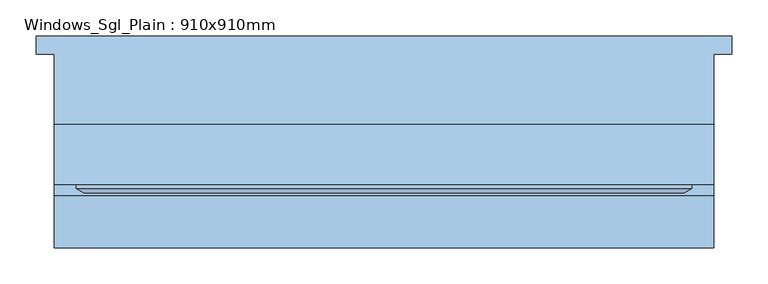
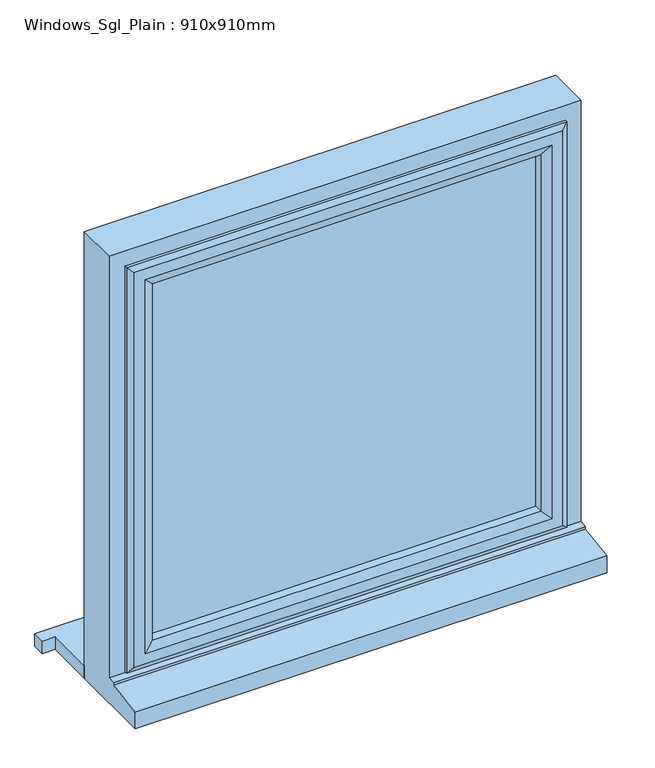
"""IFC4 building model written with IfcOpenShell, lengths in millimetres: window geometry, Windows_Sgl_Plain : 910x910mm."""

import ifcopenshell
import ifcopenshell.guid

model = None  # the IFC model being written
_history = None  # IfcOwnerHistory: only IFC2X3 demands one
_inside = {}  # id of a spatial element -> (the spatial element, [elements in it])
_under = {}  # id of a project, library or spatial element -> (it, [spatial elements below it])
_declared = {}  # id of a project -> (the project, [libraries it declares])
_typed = {}  # id of a type object -> (the type object, [elements of that type])
_made_of = {}  # id of a material, layer set ... -> (it, [elements and type objects made of it])


def new_model(schema):
    """Start an empty IFC model of exactly this schema.

    Asked for "IFC4X3", IfcOpenShell would pick the latest addendum, in which some entities
    have other attributes; the version numbers below select the first issue.
    IFC2X3 requires an IfcOwnerHistory on every rooted entity: one is made here for all.
    """
    global model, _history
    if schema == "IFC4X3":
        model = ifcopenshell.file(schema_version=(4, 3, 0, 0))
    else:
        model = ifcopenshell.file(schema=schema)
    _inside.clear()
    _under.clear()
    _declared.clear()
    _typed.clear()
    _made_of.clear()
    _history = None
    if model.schema == "IFC2X3":
        org = make("IfcOrganization", Name="unknown")
        user = make(
            "IfcPersonAndOrganization",
            ThePerson=make("IfcPerson", FamilyName="unknown"),
            TheOrganization=org,
        )
        app = make(
            "IfcApplication",
            ApplicationDeveloper=org,
            Version="unknown",
            ApplicationFullName="unknown",
            ApplicationIdentifier="unknown",
        )
        _history = make(
            "IfcOwnerHistory",
            OwningUser=user,
            OwningApplication=app,
            ChangeAction="ADDED",
            CreationDate=0,
        )
    return model


def make(cls, **values):
    """One entity of the class cls with the attributes given. An attribute that is None is left unset."""
    return model.create_entity(
        cls, **{name: value for name, value in values.items() if value is not None}
    )


def rooted(cls, **values):
    """An entity with a GlobalId (a new one), such as an element, a storey or a relation."""
    return make(cls, GlobalId=ifcopenshell.guid.new(), OwnerHistory=_history, **values)


def si_unit(unit_type, name, prefix=None):
    """IfcSIUnit, for example si_unit("LENGTHUNIT", "METRE", prefix="MILLI")."""
    return make("IfcSIUnit", UnitType=unit_type, Prefix=prefix, Name=name)


def assignment(units):
    """IfcUnitAssignment: the units of a project."""
    return None if units is None else make("IfcUnitAssignment", Units=units)


def point(xyz):
    """IfcCartesianPoint."""
    return None if xyz is None else make("IfcCartesianPoint", Coordinates=xyz)


def direction(xyz):
    """IfcDirection."""
    return None if xyz is None else make("IfcDirection", DirectionRatios=xyz)


def frame(location, z_axis=None, x_axis=None):
    """IfcAxis2Placement3D, a coordinate frame: its origin and axes. An axis left out is left unset."""
    return make(
        "IfcAxis2Placement3D",
        Location=point(location),
        Axis=direction(z_axis),
        RefDirection=direction(x_axis),
    )


def origin():
    """The frame at (0, 0, 0) with its axes left unset."""
    return frame((0.0, 0.0, 0.0))


def place(relative_to, where):
    """IfcLocalPlacement: puts the frame where relative to a parent placement (None: the world)."""
    return make(
        "IfcLocalPlacement", PlacementRelTo=relative_to, RelativePlacement=where
    )


def context(
    kind, dimensions, precision=None, world=None, true_north=None, identifier=None
):
    """IfcGeometricRepresentationContext, for example the 3D "Model" context."""
    return make(
        "IfcGeometricRepresentationContext",
        ContextIdentifier=identifier,
        ContextType=kind,
        CoordinateSpaceDimension=dimensions,
        Precision=precision,
        WorldCoordinateSystem=world,
        TrueNorth=true_north,
    )


def project(units=None, contexts=None):
    """IfcProject with its units and contexts."""
    return rooted(
        "IfcProject",
        Name="project",
        RepresentationContexts=contexts,
        UnitsInContext=assignment(units),
    )


def spatial(cls, under=None, at=None, **own):
    """A site, building, storey or space (cls), placed at a placement, below another one or the project."""
    s = rooted(cls, ObjectPlacement=at, **own)
    if under is not None:
        _under.setdefault(under.id(), (under, []))[1].append(s)
    return s


def polyline(points):
    """IfcPolyline through the points."""
    return make("IfcPolyline", Points=[point(p) for p in points])


def outline(outer, holes=None, kind="AREA"):
    """IfcArbitraryClosedProfileDef: a profile drawn as a closed curve; with holes, ...WithVoids."""
    if holes is None:
        return make("IfcArbitraryClosedProfileDef", ProfileType=kind, OuterCurve=outer)
    return make(
        "IfcArbitraryProfileDefWithVoids",
        ProfileType=kind,
        OuterCurve=outer,
        InnerCurves=holes,
    )


def extrude(swept, where, along, depth):
    """IfcExtrudedAreaSolid: the profile swept, set in the frame where, extruded along a direction by depth."""
    return make(
        "IfcExtrudedAreaSolid",
        SweptArea=swept,
        Position=where,
        ExtrudedDirection=direction(along),
        Depth=depth,
    )


def faces_of(points, faces, orient=None, outer=None):
    """IfcFace entities. A face is a list of loops; a loop is a list of indices into points, from 0.

    orient and outer hold one flag for each loop. By default every Orientation is true, the
    first loop of a face is its IfcFaceOuterBound and the others are IfcFaceBound.
    """
    made = []
    for i, loops in enumerate(faces):
        bounds = []
        for j, loop in enumerate(loops):
            is_outer = j == 0 if outer is None else outer[i][j]
            bounds.append(
                make(
                    "IfcFaceOuterBound" if is_outer else "IfcFaceBound",
                    Bound=make("IfcPolyLoop", Polygon=[points[k] for k in loop]),
                    Orientation=True if orient is None else orient[i][j],
                )
            )
        made.append(make("IfcFace", Bounds=bounds))
    return made


def faceted_brep(points, faces, orient=None, outer=None, voids=None):
    """IfcFacetedBrep: a solid bounded by flat faces; with voids (closed shells), ...WithVoids."""
    shared = [point(p) for p in points]
    hull = make("IfcClosedShell", CfsFaces=faces_of(shared, faces, orient, outer))
    if voids is None:
        return make("IfcFacetedBrep", Outer=hull)
    return make(
        "IfcFacetedBrepWithVoids",
        Outer=hull,
        Voids=[
            make(cls, CfsFaces=faces_of(shared, fs, o, b)) for cls, fs, o, b in voids
        ],
    )


def shape(context_of_items, identifier, shape_type, items):
    """IfcShapeRepresentation: the items that make up one representation, for example the "Body"."""
    return make(
        "IfcShapeRepresentation",
        ContextOfItems=context_of_items,
        RepresentationIdentifier=identifier,
        RepresentationType=shape_type,
        Items=items,
    )


def source(mapping_origin, context_of_items, identifier, shape_type, items):
    """IfcRepresentationMap: a shape defined once, which mapped items show again and again."""
    return make(
        "IfcRepresentationMap",
        MappingOrigin=mapping_origin,
        MappedRepresentation=shape(context_of_items, identifier, shape_type, items),
    )


def transform(
    local_origin,
    x_axis=None,
    y_axis=None,
    z_axis=None,
    scale=None,
    scale2=None,
    scale3=None,
    uniform=True,
):
    """IfcCartesianTransformationOperator3D, or its non-uniform kind. x_axis, y_axis, z_axis: its Axis1, 2, 3."""
    if uniform:
        return make(
            "IfcCartesianTransformationOperator3D",
            Axis1=direction(x_axis),
            Axis2=direction(y_axis),
            LocalOrigin=point(local_origin),
            Scale=scale,
            Axis3=direction(z_axis),
        )
    return make(
        "IfcCartesianTransformationOperator3DnonUniform",
        Axis1=direction(x_axis),
        Axis2=direction(y_axis),
        LocalOrigin=point(local_origin),
        Scale=scale,
        Axis3=direction(z_axis),
        Scale2=scale2,
        Scale3=scale3,
    )


def mapped(mapping_source, mapping_target):
    """IfcMappedItem: shows the shape of a source again, moved by a transform."""
    return make(
        "IfcMappedItem", MappingSource=mapping_source, MappingTarget=mapping_target
    )


def made_of(thing, what):
    """Note that an element or type object is made of a material, layer set ...; save() writes the relation."""
    if what is not None:
        _made_of.setdefault(what.id(), (what, []))[1].append(thing)
    return thing


def element(
    cls,
    number,
    at=None,
    inside=None,
    cuts=None,
    type_object=None,
    material=None,
    context=None,
    identifier="Body",
    shape_type=None,
    held_by="IfcProductDefinitionShape",
    body=None,
    shapes=None,
    **own,
):
    """One element of the class cls, such as IfcWall. Its Tag is "e" and its number.

    at: its placement. inside: the storey or other place that contains it. cuts: it is an
    opening in that element (IfcRelVoidsElement). A single representation is given by context,
    identifier, shape_type and body (its items); several are given by shapes. held_by: the class
    of the entity that holds the representations. save() writes the other relations.
    """
    e = rooted(cls, Tag="e%d" % number, ObjectPlacement=at, **own)
    if body is not None:
        shapes = [shape(context, identifier, shape_type, body)]
    if shapes is not None:
        e.Representation = make(held_by, Representations=shapes)
    if inside is not None:
        _inside.setdefault(inside.id(), (inside, []))[1].append(e)
    if cuts is not None:
        rooted(
            "IfcRelVoidsElement", RelatingBuildingElement=cuts, RelatedOpeningElement=e
        )
    if type_object is not None:
        _typed.setdefault(type_object.id(), (type_object, []))[1].append(e)
    return made_of(e, material)


def aggregate(whole, parts):
    """IfcRelAggregates: a whole, such as a stair, and the parts it consists of."""
    return rooted("IfcRelAggregates", RelatingObject=whole, RelatedObjects=parts)


def save(model, path):
    """Write the relations noted so far, then the file.

    IfcRelAggregates (storeys below a building ...), IfcRelContainedInSpatialStructure (elements
    in a storey), IfcRelDefinesByType, IfcRelAssociatesMaterial and IfcRelDeclares: one each for
    every whole, place, type object, material and project.
    """
    for whole, parts in _under.values():
        aggregate(whole, parts)
    for where, things in _inside.values():
        rooted(
            "IfcRelContainedInSpatialStructure",
            RelatedElements=things,
            RelatingStructure=where,
        )
    for kind, things in _typed.values():
        rooted("IfcRelDefinesByType", RelatedObjects=things, RelatingType=kind)
    for what, things in _made_of.values():
        rooted("IfcRelAssociatesMaterial", RelatedObjects=things, RelatingMaterial=what)
    for by, libraries in _declared.values():
        rooted("IfcRelDeclares", RelatingContext=by, RelatedDefinitions=libraries)
    model.write(path)


def windows_sgl_plain_910x910mm_d8acfbc0(model_context):
    return source(origin(), model_context, "Body", "SolidModel", [
        extrude(outline(polyline([(-480.0, 131.5434322), (480.0, 131.5434322), (480.0, 106.5434322), (455.0, 106.5434322), (455.0, 9.5434322), (-455.0, 9.5434322), (-455.0, 106.5434322), (-480.0, 106.5434322), (-480.0, 131.5434322)])), frame((0.0, 0.0, 1200.0), z_axis=(0.0, 0.0, 1.0), x_axis=(1.0, 0.0, 0.0)), (0.0, 0.0, 1.0), 25.0),
        faceted_brep([(-455.0, 9.5434322, 1200.0), (-455.0, 9.5434322, 2110.0), (455.0, 9.5434322, 2110.0), (455.0, 9.5434322, 1200.0), (-395.0, 9.5434322, 2050.0), (-395.0, 9.5434322, 1275.0), (395.0, 9.5434322, 1275.0), (395.0, 9.5434322, 2050.0), (-455.0, -160.9565678, 1200.0), (-455.0, -160.9565678, 1233.8088847), (-455.0, -88.4565678, 1244.7449676), (-455.0, -88.4565678, 1249.68767), (-455.0, -73.4565678, 1251.0), (-455.0, -73.4565678, 2110.0), (455.0, -73.4565678, 1251.0), (455.0, -73.4565678, 2110.0), (-415.0, -73.4565678, 2070.0), (415.0, -73.4565678, 2070.0), (415.0, -73.4565678, 1263.0), (-415.0, -73.4565678, 1263.0), (-415.0, -8.4565678, 1263.0), (-415.0, -8.4565678, 2070.0), (415.0, -8.4565678, 1263.0), (415.0, -8.4565678, 2070.0), (-395.0, -8.4565678, 2050.0), (395.0, -8.4565678, 2050.0), (395.0, -8.4565678, 1275.0), (-395.0, -8.4565678, 1275.0), (455.0, -88.4565678, 1249.68767), (455.0, -88.4565678, 1244.7449676), (455.0, -160.9565678, 1233.8088847), (455.0, -160.9565678, 1200.0)], [[[0, 1, 2, 3], [4, 5, 6, 7]], [[0, 8, 9, 10, 11, 12, 13, 1]], [[12, 14, 15, 13], [16, 17, 18, 19]], [[19, 20, 21, 16]], [[21, 20, 22, 23], [24, 25, 26, 27]], [[24, 27, 5, 4]], [[1, 13, 15, 2]], [[16, 21, 23, 17]], [[7, 25, 24, 4]], [[14, 28, 29, 30, 31, 3, 2, 15]], [[17, 23, 22, 18]], [[7, 6, 26, 25]], [[31, 8, 0, 3]], [[30, 9, 8, 31]], [[29, 10, 9, 30]], [[28, 11, 10, 29]], [[14, 12, 11, 28]], [[20, 19, 18, 22]], [[5, 27, 26, 6]]]),
        extrude(outline(polyline([(385.0, -37.4565678), (385.0, -61.4565678), (-385.0, -61.4565678), (-385.0, -37.4565678), (385.0, -37.4565678)])), frame((0.0, 0.0, 1293.0), z_axis=(0.0, 0.0, 1.0), x_axis=(1.0, 0.0, 0.0)), (0.0, 0.0, 1.0), 747.0),
        faceted_brep([(-425.0, -73.4565678, 2080.0), (-425.0, -73.4565678, 1253.0), (-425.0, -79.2300705, 1253.0), (-425.0, -79.2300705, 2080.0), (-415.0, -8.4565678, 2070.0), (-415.0, -8.4565678, 1263.0), (-415.0, -73.4565678, 1263.0), (-415.0, -73.4565678, 2070.0), (-375.0, -22.9494677, 2030.0), (-375.0, -22.9494677, 1303.0), (-385.1480377, -8.4565678, 1292.8519623), (-385.1480377, -8.4565678, 2040.1480377), (-375.0, -37.4565678, 2030.0), (-375.0, -37.4565678, 1303.0), (-385.0, -61.4565678, 2040.0), (-385.0, -61.4565678, 1293.0), (-385.0, -37.4565678, 1293.0), (-385.0, -37.4565678, 2040.0), (-375.0, -79.2300705, 2030.0), (-375.0, -79.2300705, 1303.0), (-375.0, -61.4565678, 1303.0), (-375.0, -61.4565678, 2030.0), (-392.4457548, -85.0035732, 2047.4457548), (-392.4457548, -85.0035732, 1285.5542452), (-414.2153903, -85.0035732, 1263.7846097), (-414.2153903, -85.0035732, 2069.2153903), (425.0, -73.4565678, 1253.0), (425.0, -79.2300705, 1253.0), (415.0, -8.4565678, 1263.0), (415.0, -73.4565678, 1263.0), (375.0, -22.9494677, 1303.0), (385.1480377, -8.4565678, 1292.8519623), (375.0, -37.4565678, 1303.0), (385.0, -61.4565678, 1293.0), (385.0, -37.4565678, 1293.0), (375.0, -79.2300705, 1303.0), (375.0, -61.4565678, 1303.0), (392.4457548, -85.0035732, 1285.5542452), (414.2153903, -85.0035732, 1263.7846097), (425.0, -73.4565678, 2080.0), (425.0, -79.2300705, 2080.0), (415.0, -8.4565678, 2070.0), (415.0, -73.4565678, 2070.0), (375.0, -22.9494677, 2030.0), (385.1480377, -8.4565678, 2040.1480377), (375.0, -37.4565678, 2030.0), (385.0, -61.4565678, 2040.0), (385.0, -37.4565678, 2040.0), (375.0, -79.2300705, 2030.0), (375.0, -61.4565678, 2030.0), (392.4457548, -85.0035732, 2047.4457548), (414.2153903, -85.0035732, 2069.2153903)], [[[0, 1, 2, 3]], [[4, 5, 6, 7]], [[8, 9, 10, 11]], [[12, 13, 9, 8]], [[14, 15, 16, 17]], [[18, 19, 20, 21]], [[22, 23, 19, 18]], [[3, 2, 24, 25]], [[1, 26, 27, 2]], [[5, 28, 29, 6]], [[9, 30, 31, 10]], [[13, 32, 30, 9]], [[15, 33, 34, 16]], [[19, 35, 36, 20]], [[23, 37, 35, 19]], [[2, 27, 38, 24]], [[26, 39, 40, 27]], [[28, 41, 42, 29]], [[30, 43, 44, 31]], [[32, 45, 43, 30]], [[33, 46, 47, 34]], [[35, 48, 49, 36]], [[37, 50, 48, 35]], [[27, 40, 51, 38]], [[39, 0, 3, 40]], [[1, 0, 39, 26], [7, 6, 29, 42]], [[41, 4, 7, 42]], [[5, 4, 41, 28], [11, 10, 31, 44]], [[43, 8, 11, 44]], [[45, 12, 8, 43]], [[17, 16, 34, 47], [13, 12, 45, 32]], [[46, 14, 17, 47]], [[15, 14, 46, 33], [21, 20, 36, 49]], [[48, 18, 21, 49]], [[50, 22, 18, 48]], [[25, 24, 38, 51], [23, 22, 50, 37]], [[40, 3, 25, 51]]]),
    ])


if __name__ == "__main__":
    model = new_model("IFC4")
    model_context = context("Model", 3, world=origin())
    ifc_project = project(units=[si_unit("LENGTHUNIT", "METRE", prefix="MILLI")], contexts=[model_context])
    site = spatial("IfcSite", under=ifc_project)
    building = spatial("IfcBuilding", under=site)
    placement = place(None, origin())
    windows_sgl_plain_910x910mm_shape = windows_sgl_plain_910x910mm_d8acfbc0(model_context)
    element("IfcWindow", 1, ObjectType="Windows_Sgl_Plain : 910x910mm", at=placement, inside=building, context=model_context, shape_type="MappedRepresentation", body=[
        mapped(windows_sgl_plain_910x910mm_shape, transform((0.0, 0.0, 0.0), x_axis=(1.0, 0.0, 0.0), y_axis=(0.0, 1.0, 0.0), z_axis=(0.0, 0.0, 1.0))),
    ])
    save(model, "model.ifc")

# Revit data of these elements
# Type "Windows_Sgl_Plain : 910x910mm"
#   Type Mark = "44"
#   Operation = "SinglePanel"
#   Construction Type Id = "SGL"
#   Manufacturer = "Revit"
#   Keynote = "L10"
#   Analytic Construction = "Large single-glazed windows"
#   Wrap Layers (Ext) from Ext = 102.5 mm
#   Wrap Layers (Int) from Ext = 177.5 mm
#   Window Board Projection = 25 mm
#   Window Board Extension = 25 mm
#   Visual Light Transmittance = 0.9
#   Solar Heat Gain Coefficient = 0.86
#   Rough Width = 910 mm
#   Rough Height = 910 mm
#   Height = 910 mm
#   Width = 910 mm
#   Heat Transfer Coefficient (U) = 5.5617 W/(m²·K)
#   Glazing Thickness = 24 mm
#   FrameOffset - External = 50 mm
#   Frame Depth = 65 mm
#   Default Head Height = 2110 mm
#   Cill Depth = 87.5 mm
#   Cavity Closer Width = 50 mm
#   Cavity Closer Offset from Ext = 102.5 mm
#   Cavity Closer Depth = 85 mm
#   Define Thermal Properties by = 1
#   Vis - Cavity Closers = yes
#   Define Thermal Properties by = 1
#   Material Trim = Window Frame
#   Material Glass = Glass
#   Material Frame = Window Frame
#   Wall Closure = (empty or 0)
# Element 1 (IfcWindow, "Windows_Sgl_Plain : 910x910mm")
#   Materials on its faces: "Window Frame", "Glass"
# Materials
#   "Window Frame": class "Miscellaneous", colour RGB 249 249 249, transparency 0, Keynote = "L10", Cost = 0
#   "Glass": class "Glass", colour RGB 0 128 192, transparency 0.9, Description = "Soda Lime Glass", Cost = 0
